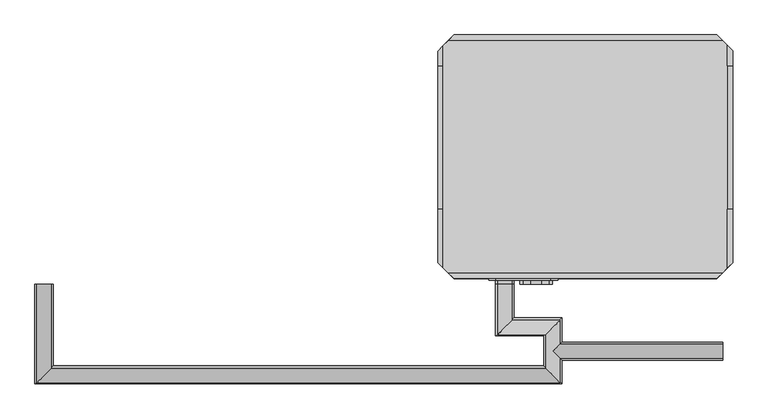
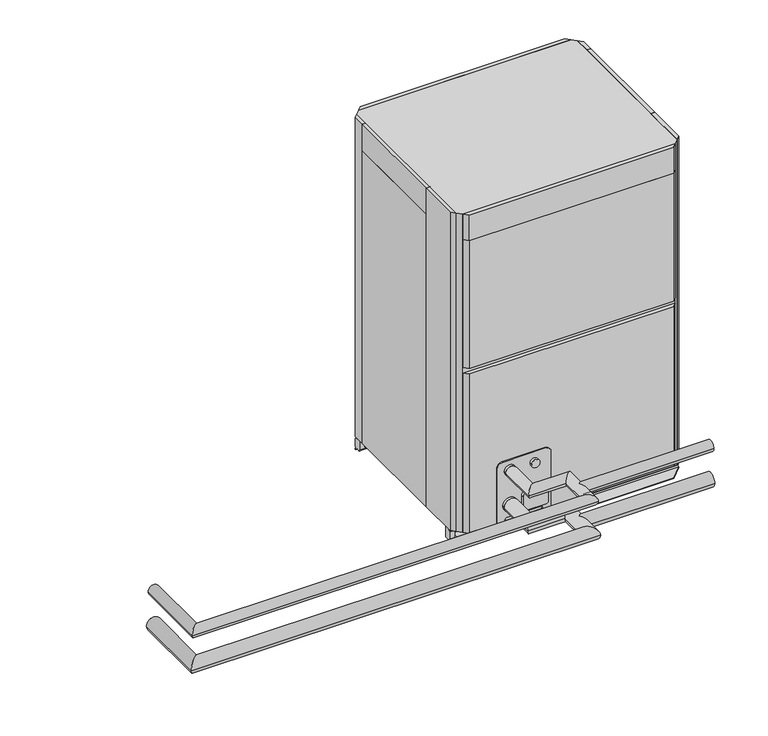
# IFC4 building model written with IfcOpenShell, lengths in millimetres: proxy geometry, PURY-P168-288_YSJMU_Heat_Recovery_460V : PURY-P192YSJMU-A(-BS)_460V.
# Revit data of these elements (continued)
# Type "PURY-P168-288_YSJMU_Heat_Recovery_460V : PURY-P192YSJMU-A(-BS)_460V" (continued)
#   Refrigerant Pipe diameter (high pressure) = 22.225 mm
#   Phase = 3
#   Outdoor Unit2-Width = 920 mm
#   Outdoor Unit1-Width = 1750 mm
#   Offset = 30 mm
#   Hertz = 60
#   Height = 1650 mm
#   Depth = 760 mm
#   Apparent Load = 0 VA
#   Number of Poles = 2
#   Load Classification = Other
#   External Material = Pre-coated Galvanized-steel Sheets
#   External Finish = Pre-coated Galvanized-steel Sheets
#   Air Outlet Unit Material = Metal Grille
#   Air Inlet Unit Material = Grille
#   Type Comments = ""
#   Description = (empty or 0)
#   Default Elevation = 0
# Element 1 (IfcBuildingElementProxy, "PURY-P168-288_YSJMU_Heat_Recovery_460V : PURY-P192YSJMU-A(-BS)_460V")
#   Materials on its faces: "Pre-coated Galvanized-steel Sheets", "Grille", "Metal Grille"
# Materials
#   "Pre-coated Galvanized-steel Sheets": class "Metal", colour RGB 189 187 185, transparency 0
#   "Metal Grille": class "Metal", colour RGB 10 10 10, transparency 0
#   "Grille": class "Miscellaneous", colour RGB 0 0 0, transparency 0
